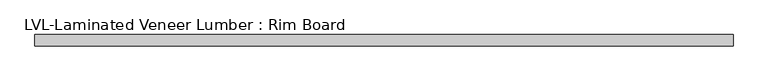
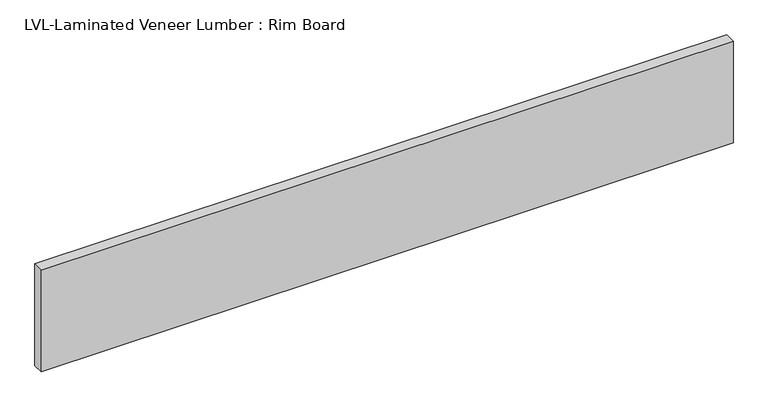
"""IFC4 building model written with IfcOpenShell, lengths in millimetres: beam geometry, LVL-Laminated Veneer Lumber : Rim Board."""

from ifc_helpers import new_model, si_unit, frame, origin, place, context, project, spatial, polyline, outline, extrude, source, transform, mapped, element, save


def lvl_laminated_veneer_lumber_rim_board_571f3e0e(model_context):
    return source(origin(), model_context, "Body", "SweptSolid", [
        extrude(outline(polyline([(971.55, 15.875), (971.55, -15.875), (-971.55, -15.875), (-971.55, 15.875), (971.55, 15.875)])), frame((0.0, 0.0, -150.8125), z_axis=(0.0, 0.0, 1.0), x_axis=(1.0, 0.0, 0.0)), (0.0, 0.0, 1.0), 301.625),
    ])


if __name__ == "__main__":
    model = new_model("IFC4")
    model_context = context("Model", 3, world=origin())
    ifc_project = project(units=[si_unit("LENGTHUNIT", "METRE", prefix="MILLI")], contexts=[model_context])
    site = spatial("IfcSite", under=ifc_project)
    building = spatial("IfcBuilding", under=site)
    placement = place(None, origin())
    lvl_laminated_veneer_lumber_rim_board_shape = lvl_laminated_veneer_lumber_rim_board_571f3e0e(model_context)
    element("IfcBeam", 1, ObjectType="LVL-Laminated Veneer Lumber : Rim Board", at=placement, inside=building, context=model_context, shape_type="MappedRepresentation", body=[
        mapped(lvl_laminated_veneer_lumber_rim_board_shape, transform((0.0, 0.0, 0.0), x_axis=(1.0, 0.0, 0.0), y_axis=(0.0, 1.0, 0.0), z_axis=(0.0, 0.0, 1.0))),
    ])
    save(model, "model.ifc")

# Revit data of these elements
# Type "LVL-Laminated Veneer Lumber : Rim Board"
#   Assembly Code = "B10"
#   Cost = 4.6
#   Length [instance default] = 5' - 0"
#   b = 0' - 1 1/4"
#   d = 0' - 11 7/8"
#   Structural Material [instance default] = Softwood, Lumber
# Element 1 (IfcBeam, "LVL-Laminated Veneer Lumber : Rim Board")
#   Structural Material = Douglas Fir #2
#   Materials on its faces: "Douglas Fir #2"
# Materials
#   "Softwood, Lumber": class "Wood", colour RGB 223 192 134, transparency 0, Description = "Pinus Echinata", Cost = 0
#   "Douglas Fir #2": class "Wood", colour RGB 223 192 134, transparency 0, Description = "Pinus Echinata", Cost = 0
